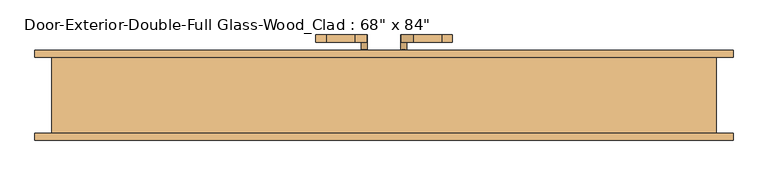
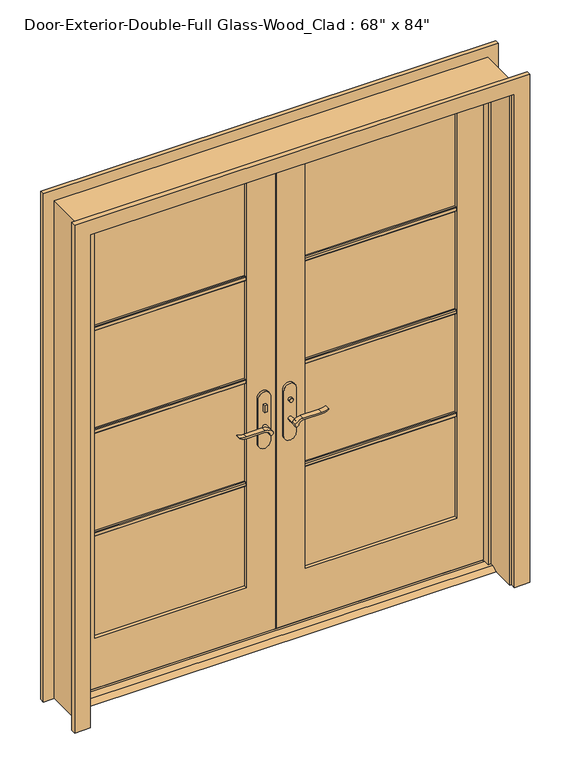
"""IFC4 building model written with IfcOpenShell, lengths in millimetres: door geometry."""

from ifc_helpers import new_model, si_unit, point, frame, frame_2d, origin, place, context, project, spatial, polyline, circle_curve, trimmed, segment, composite_curve, outline, extrude, faceted_brep, source, transform, mapped, element, save


def door_f342fe49(model_context):
    return source(origin(), model_context, "Body", "SolidModel", [
        extrude(outline(polyline([(19.05, 12.7), (53.975, 12.7), (79.375, 0.0), (-6.35, 0.0), (19.05, 12.7)])), frame((-863.6, 0.0, 0.0), z_axis=(1.0, 0.0, 0.0), x_axis=(0.0, 1.0, 0.0)), (0.0, 0.0, 1.0), 1727.2),
        extrude(outline(polyline([(-47.4019111, 43.5), (-57.4019111, 43.5), (-57.4019111, 53.5), (-47.4019111, 53.5), (-47.4019111, 43.5)])), frame((0.0, 0.0, 981.9), z_axis=(0.0, 0.0, 1.0), x_axis=(1.0, 0.0, 0.0)), (0.0, 0.0, 1.0), 30.0),
        extrude(outline(composite_curve([segment(trimmed(circle_curve(frame_2d((996.9, -52.4019111)), 8.0), [point((996.9, -60.4019111))], [point((996.9, -44.4019111))], False, "CARTESIAN"), True, "CONTINUOUS"), segment(trimmed(circle_curve(frame_2d((996.9, -52.4019111)), 8.0), [point((996.9, -44.4019111))], [point((996.9, -60.4019111))], False, "CARTESIAN"), True, "CONTINUOUS")], self_intersect=False)), frame((0.0, 108.425, 0.0), z_axis=(0.0, 1.0, 0.0), x_axis=(0.0, 0.0, 1.0)), (0.0, 0.0, 1.0), 10.0),
        extrude(outline(composite_curve([segment(trimmed(circle_curve(frame_2d((897.1555521, -76.0694241)), 37.2832219), [point((919.0523287, -45.8937749))], [point((934.4, -77.7693445))], False, "CARTESIAN"), True, "CONTINUOUS"), segment(polyline([(934.4, -77.7693445), (934.4, -154.045502)]), True, "CONTINUOUS"), segment(trimmed(circle_curve(frame_2d((1017.6850638, -153.9791202)), 83.2850902), [point((934.4, -154.045502))], [point((939.4, -182.4019111))], True, "CARTESIAN"), True, "CONTINUOUS"), segment(polyline([(939.4, -182.4019111), (936.6135558, -182.4019111)]), True, "CONTINUOUS"), segment(trimmed(circle_curve(frame_2d((986.6709207, -150.4622499)), 59.3791355), [point((936.6135558, -182.4019111))], [point((927.4, -154.045502))], False, "CARTESIAN"), True, "CONTINUOUS"), segment(polyline([(927.4, -154.045502), (927.4, -77.7881013)]), True, "CONTINUOUS"), segment(trimmed(circle_curve(frame_2d((909.2738613, -77.7881013)), 18.1261387), [point((927.4, -77.7881013))], [point((914.4, -60.4019111))], True, "CARTESIAN"), True, "CONTINUOUS"), segment(trimmed(circle_curve(frame_2d((914.4, -52.4019111)), 8.0), [point((914.4, -60.4019111))], [point((919.0523287, -45.8937749))], False, "CARTESIAN"), True, "CONTINUOUS")], self_intersect=False)), frame((0.0, 3.5, 0.0), z_axis=(0.0, 1.0, 0.0), x_axis=(0.0, 0.0, 1.0)), (0.0, 0.0, 1.0), 20.0),
        extrude(outline(composite_curve([segment(trimmed(circle_curve(frame_2d((914.4, -52.4019111)), 8.0), [point((914.3999903, -60.4019111))], [point((919.0523287, -45.8937749))], False, "CARTESIAN"), True, "CONTINUOUS"), segment(trimmed(circle_curve(frame_2d((897.1555521, -76.0694241)), 37.2832219), [point((919.0523287, -45.8937749))], [point((934.4, -77.7693445))], False, "CARTESIAN"), True, "CONTINUOUS"), segment(polyline([(934.4, -77.7693445), (934.4, -154.045502)]), True, "CONTINUOUS"), segment(trimmed(circle_curve(frame_2d((1017.6850638, -153.9791202)), 83.2850902), [point((934.4, -154.045502))], [point((939.4, -182.4019111))], True, "CARTESIAN"), True, "CONTINUOUS"), segment(polyline([(939.4, -182.4019111), (936.6135558, -182.4019111)]), True, "CONTINUOUS"), segment(trimmed(circle_curve(frame_2d((986.6709207, -150.4622499)), 59.3791355), [point((936.6135558, -182.4019111))], [point((927.4, -154.045502))], False, "CARTESIAN"), True, "CONTINUOUS"), segment(polyline([(927.4, -154.045502), (927.4, -77.788099)]), True, "CONTINUOUS"), segment(trimmed(circle_curve(frame_2d((909.2738682, -77.788099)), 18.1261318), [point((927.4, -77.788099))], [point((914.3999903, -60.4019111))], True, "CARTESIAN"), True, "CONTINUOUS")], self_intersect=False)), frame((0.0, 138.425, 0.0), z_axis=(0.0, 1.0, 0.0), x_axis=(0.0, 0.0, 1.0)), (0.0, 0.0, 1.0), 20.0),
        extrude(outline(composite_curve([segment(trimmed(circle_curve(frame_2d((914.4, -52.4019111)), 8.0), [point((914.4, -60.4019111))], [point((914.4, -44.4019111))], False, "CARTESIAN"), True, "CONTINUOUS"), segment(trimmed(circle_curve(frame_2d((914.4, -52.4019111)), 8.0), [point((914.4, -44.4019111))], [point((914.4, -60.4019111))], False, "CARTESIAN"), True, "CONTINUOUS")], self_intersect=False)), frame((0.0, 23.5, 0.0), z_axis=(0.0, 1.0, 0.0), x_axis=(0.0, 0.0, 1.0)), (0.0, 0.0, 1.0), 30.0),
        extrude(outline(composite_curve([segment(trimmed(circle_curve(frame_2d((914.4, -52.4019111)), 8.0), [point((914.4, -60.4019111))], [point((914.4, -44.4019111))], False, "CARTESIAN"), True, "CONTINUOUS"), segment(trimmed(circle_curve(frame_2d((914.4, -52.4019111)), 8.0), [point((914.4, -44.4019111))], [point((914.4, -60.4019111))], False, "CARTESIAN"), True, "CONTINUOUS")], self_intersect=False)), frame((0.0, 108.425, 0.0), z_axis=(0.0, 1.0, 0.0), x_axis=(0.0, 0.0, 1.0)), (0.0, 0.0, 1.0), 30.0),
        extrude(outline(composite_curve([segment(polyline([(844.4, -27.4019111), (1039.4, -27.4019111)]), True, "CONTINUOUS"), segment(trimmed(circle_curve(frame_2d((1039.4, -52.4019111)), 25.0), [point((1039.4, -27.4019111))], [point((1039.4, -77.4019111))], False, "CARTESIAN"), True, "CONTINUOUS"), segment(polyline([(1039.4, -77.4019111), (844.4, -77.4019111)]), True, "CONTINUOUS"), segment(trimmed(circle_curve(frame_2d((844.4, -52.4019111)), 25.0), [point((844.4, -77.4019111))], [point((844.4, -27.4019111))], False, "CARTESIAN"), True, "CONTINUOUS")], self_intersect=False)), frame((0.0, 53.5, 0.0), z_axis=(0.0, 1.0, 0.0), x_axis=(0.0, 0.0, 1.0)), (0.0, 0.0, 1.0), 10.0),
        extrude(outline(composite_curve([segment(polyline([(844.4, -27.4019111), (1039.4, -27.4019111)]), True, "CONTINUOUS"), segment(trimmed(circle_curve(frame_2d((1039.4, -52.4019111)), 25.0), [point((1039.4, -27.4019111))], [point((1039.4, -77.4019111))], False, "CARTESIAN"), True, "CONTINUOUS"), segment(polyline([(1039.4, -77.4019111), (844.4, -77.4019111)]), True, "CONTINUOUS"), segment(trimmed(circle_curve(frame_2d((844.4, -52.4019111)), 25.0), [point((844.4, -77.4019111))], [point((844.4, -27.4019111))], False, "CARTESIAN"), True, "CONTINUOUS")], self_intersect=False)), frame((0.0, 98.425, 0.0), z_axis=(0.0, 1.0, 0.0), x_axis=(0.0, 0.0, 1.0)), (0.0, 0.0, 1.0), 10.0),
        extrude(outline(polyline([(47.3875, 118.425), (57.3875, 118.425), (57.3875, 108.425), (47.3875, 108.425), (47.3875, 118.425)])), frame((0.0, 0.0, 981.9), z_axis=(0.0, 0.0, 1.0), x_axis=(1.0, 0.0, 0.0)), (0.0, 0.0, 1.0), 30.0),
        extrude(outline(composite_curve([segment(trimmed(circle_curve(frame_2d((996.9, 52.3875)), 8.0), [point((996.9, 60.3875))], [point((996.9, 44.3875))], False, "CARTESIAN"), True, "CONTINUOUS"), segment(trimmed(circle_curve(frame_2d((996.9, 52.3875)), 8.0), [point((996.9, 44.3875))], [point((996.9, 60.3875))], False, "CARTESIAN"), True, "CONTINUOUS")], self_intersect=False)), frame((0.0, 43.5, 0.0), z_axis=(0.0, 1.0, 0.0), x_axis=(0.0, 0.0, 1.0)), (0.0, 0.0, 1.0), 10.0),
        extrude(outline(composite_curve([segment(trimmed(circle_curve(frame_2d((914.4, 52.3875)), 8.0), [point((919.0523287, 45.8793637))], [point((914.4, 60.3875))], False, "CARTESIAN"), True, "CONTINUOUS"), segment(trimmed(circle_curve(frame_2d((909.2738613, 77.7736901)), 18.1261387), [point((914.4, 60.3875))], [point((927.4, 77.7736901))], True, "CARTESIAN"), True, "CONTINUOUS"), segment(polyline([(927.4, 77.7736901), (927.4, 154.0310909)]), True, "CONTINUOUS"), segment(trimmed(circle_curve(frame_2d((986.6709207, 150.4478388)), 59.3791355), [point((927.4, 154.0310909))], [point((936.6135558, 182.3875))], False, "CARTESIAN"), True, "CONTINUOUS"), segment(polyline([(936.6135558, 182.3875), (939.4, 182.3875)]), True, "CONTINUOUS"), segment(trimmed(circle_curve(frame_2d((1017.6850638, 153.9647091)), 83.2850902), [point((939.4, 182.3875))], [point((934.4, 154.0310909))], True, "CARTESIAN"), True, "CONTINUOUS"), segment(polyline([(934.4, 154.0310909), (934.4, 77.7549333)]), True, "CONTINUOUS"), segment(trimmed(circle_curve(frame_2d((897.1555521, 76.0550129)), 37.2832219), [point((934.4, 77.7549333))], [point((919.0523287, 45.8793637))], False, "CARTESIAN"), True, "CONTINUOUS")], self_intersect=False)), frame((0.0, 138.425, 0.0), z_axis=(0.0, 1.0, 0.0), x_axis=(0.0, 0.0, 1.0)), (0.0, 0.0, 1.0), 20.0),
        extrude(outline(composite_curve([segment(trimmed(circle_curve(frame_2d((909.2738682, 77.7736878)), 18.1261318), [point((914.3999903, 60.3875))], [point((927.4, 77.7736878))], True, "CARTESIAN"), True, "CONTINUOUS"), segment(polyline([(927.4, 77.7736878), (927.4, 154.0310909)]), True, "CONTINUOUS"), segment(trimmed(circle_curve(frame_2d((986.6709207, 150.4478388)), 59.3791355), [point((927.4, 154.0310909))], [point((936.6135558, 182.3875))], False, "CARTESIAN"), True, "CONTINUOUS"), segment(polyline([(936.6135558, 182.3875), (939.4, 182.3875)]), True, "CONTINUOUS"), segment(trimmed(circle_curve(frame_2d((1017.6850638, 153.9647091)), 83.2850902), [point((939.4, 182.3875))], [point((934.4, 154.0310909))], True, "CARTESIAN"), True, "CONTINUOUS"), segment(polyline([(934.4, 154.0310909), (934.4, 77.7549333)]), True, "CONTINUOUS"), segment(trimmed(circle_curve(frame_2d((897.1555521, 76.0550129)), 37.2832219), [point((934.4, 77.7549333))], [point((919.0523287, 45.8793637))], False, "CARTESIAN"), True, "CONTINUOUS"), segment(trimmed(circle_curve(frame_2d((914.4, 52.3875)), 8.0), [point((919.0523287, 45.8793637))], [point((914.3999903, 60.3875))], False, "CARTESIAN"), True, "CONTINUOUS")], self_intersect=False)), frame((0.0, 3.5, 0.0), z_axis=(0.0, 1.0, 0.0), x_axis=(0.0, 0.0, 1.0)), (0.0, 0.0, 1.0), 20.0),
        extrude(outline(composite_curve([segment(trimmed(circle_curve(frame_2d((914.4, 52.3875)), 8.0), [point((914.4, 60.3875))], [point((914.4, 44.3875))], False, "CARTESIAN"), True, "CONTINUOUS"), segment(trimmed(circle_curve(frame_2d((914.4, 52.3875)), 8.0), [point((914.4, 44.3875))], [point((914.4, 60.3875))], False, "CARTESIAN"), True, "CONTINUOUS")], self_intersect=False)), frame((0.0, 108.425, 0.0), z_axis=(0.0, 1.0, 0.0), x_axis=(0.0, 0.0, 1.0)), (0.0, 0.0, 1.0), 30.0),
        extrude(outline(composite_curve([segment(trimmed(circle_curve(frame_2d((914.4, 52.3875)), 8.0), [point((914.4, 60.3875))], [point((914.4, 44.3875))], False, "CARTESIAN"), True, "CONTINUOUS"), segment(trimmed(circle_curve(frame_2d((914.4, 52.3875)), 8.0), [point((914.4, 44.3875))], [point((914.4, 60.3875))], False, "CARTESIAN"), True, "CONTINUOUS")], self_intersect=False)), frame((0.0, 23.5, 0.0), z_axis=(0.0, 1.0, 0.0), x_axis=(0.0, 0.0, 1.0)), (0.0, 0.0, 1.0), 30.0),
        extrude(outline(composite_curve([segment(trimmed(circle_curve(frame_2d((844.4, 52.3875)), 25.0), [point((844.4, 27.3875))], [point((844.4, 77.3875))], False, "CARTESIAN"), True, "CONTINUOUS"), segment(polyline([(844.4, 77.3875), (1039.4, 77.3875)]), True, "CONTINUOUS"), segment(trimmed(circle_curve(frame_2d((1039.4, 52.3875)), 25.0), [point((1039.4, 77.3875))], [point((1039.4, 27.3875))], False, "CARTESIAN"), True, "CONTINUOUS"), segment(polyline([(1039.4, 27.3875), (844.4, 27.3875)]), True, "CONTINUOUS")], self_intersect=False)), frame((0.0, 98.425, 0.0), z_axis=(0.0, 1.0, 0.0), x_axis=(0.0, 0.0, 1.0)), (0.0, 0.0, 1.0), 10.0),
        extrude(outline(composite_curve([segment(trimmed(circle_curve(frame_2d((844.4, 52.3875)), 25.0), [point((844.4, 27.3875))], [point((844.4, 77.3875))], False, "CARTESIAN"), True, "CONTINUOUS"), segment(polyline([(844.4, 77.3875), (1039.4, 77.3875)]), True, "CONTINUOUS"), segment(trimmed(circle_curve(frame_2d((1039.4, 52.3875)), 25.0), [point((1039.4, 77.3875))], [point((1039.4, 27.3875))], False, "CARTESIAN"), True, "CONTINUOUS"), segment(polyline([(1039.4, 27.3875), (844.4, 27.3875)]), True, "CONTINUOUS")], self_intersect=False)), frame((0.0, 53.5, 0.0), z_axis=(0.0, 1.0, 0.0), x_axis=(0.0, 0.0, 1.0)), (0.0, 0.0, 1.0), 10.0),
        extrude(outline(polyline([(77.47, 1578.371875), (77.47, 1559.321875), (71.12, 1559.321875), (67.945, 1562.496875), (67.945, 1575.196875), (71.12, 1578.371875), (77.47, 1578.371875)])), frame((120.65, 0.0, 0.0), z_axis=(1.0, 0.0, 0.0), x_axis=(0.0, 1.0, 0.0)), (0.0, 0.0, 1.0), 622.3),
        extrude(outline(polyline([(77.47, 1132.68125), (77.47, 1113.63125), (71.12, 1113.63125), (67.945, 1116.80625), (67.945, 1129.50625), (71.12, 1132.68125), (77.47, 1132.68125)])), frame((120.65, 0.0, 0.0), z_axis=(1.0, 0.0, 0.0), x_axis=(0.0, 1.0, 0.0)), (0.0, 0.0, 1.0), 622.3),
        extrude(outline(polyline([(77.47, 686.990625), (77.47, 667.940625), (71.12, 667.940625), (67.945, 671.115625), (67.945, 683.815625), (71.12, 686.990625), (77.47, 686.990625)])), frame((120.65, 0.0, 0.0), z_axis=(1.0, 0.0, 0.0), x_axis=(0.0, 1.0, 0.0)), (0.0, 0.0, 1.0), 622.3),
        extrude(outline(polyline([(84.455, 1578.371875), (90.805, 1578.371875), (93.98, 1575.196875), (93.98, 1562.496875), (90.805, 1559.321875), (84.455, 1559.321875), (84.455, 1578.371875)])), frame((-742.95, 0.0, 0.0), z_axis=(1.0, 0.0, 0.0), x_axis=(0.0, 1.0, 0.0)), (0.0, 0.0, 1.0), 622.3),
        extrude(outline(polyline([(84.455, 1132.68125), (90.805, 1132.68125), (93.98, 1129.50625), (93.98, 1116.80625), (90.805, 1113.63125), (84.455, 1113.63125), (84.455, 1132.68125)])), frame((-742.95, 0.0, 0.0), z_axis=(1.0, 0.0, 0.0), x_axis=(0.0, 1.0, 0.0)), (0.0, 0.0, 1.0), 622.3),
        extrude(outline(polyline([(84.455, 686.990625), (90.805, 686.990625), (93.98, 683.815625), (93.98, 671.115625), (90.805, 667.940625), (84.455, 667.940625), (84.455, 686.990625)])), frame((-742.95, 0.0, 0.0), z_axis=(1.0, 0.0, 0.0), x_axis=(0.0, 1.0, 0.0)), (0.0, 0.0, 1.0), 622.3),
        extrude(outline(polyline([(84.455, 1578.371875), (90.805, 1578.371875), (93.98, 1575.196875), (93.98, 1562.496875), (90.805, 1559.321875), (84.455, 1559.321875), (84.455, 1578.371875)])), frame((120.65, 0.0, 0.0), z_axis=(1.0, 0.0, 0.0), x_axis=(0.0, 1.0, 0.0)), (0.0, 0.0, 1.0), 622.3),
        extrude(outline(polyline([(84.455, 1132.68125), (90.805, 1132.68125), (93.98, 1129.50625), (93.98, 1116.80625), (90.805, 1113.63125), (84.455, 1113.63125), (84.455, 1132.68125)])), frame((120.65, 0.0, 0.0), z_axis=(1.0, 0.0, 0.0), x_axis=(0.0, 1.0, 0.0)), (0.0, 0.0, 1.0), 622.3),
        extrude(outline(polyline([(84.455, 686.990625), (90.805, 686.990625), (93.98, 683.815625), (93.98, 671.115625), (90.805, 667.940625), (84.455, 667.940625), (84.455, 686.990625)])), frame((120.65, 0.0, 0.0), z_axis=(1.0, 0.0, 0.0), x_axis=(0.0, 1.0, 0.0)), (0.0, 0.0, 1.0), 622.3),
        extrude(outline(polyline([(77.47, 1578.371875), (77.47, 1559.321875), (71.12, 1559.321875), (67.945, 1562.496875), (67.945, 1575.196875), (71.12, 1578.371875), (77.47, 1578.371875)])), frame((-742.95, 0.0, 0.0), z_axis=(1.0, 0.0, 0.0), x_axis=(0.0, 1.0, 0.0)), (0.0, 0.0, 1.0), 622.3),
        extrude(outline(polyline([(77.47, 1132.68125), (77.47, 1113.63125), (71.12, 1113.63125), (67.945, 1116.80625), (67.945, 1129.50625), (71.12, 1132.68125), (77.47, 1132.68125)])), frame((-742.95, 0.0, 0.0), z_axis=(1.0, 0.0, 0.0), x_axis=(0.0, 1.0, 0.0)), (0.0, 0.0, 1.0), 622.3),
        extrude(outline(polyline([(77.47, 686.990625), (77.47, 667.940625), (71.12, 667.940625), (67.945, 671.115625), (67.945, 683.815625), (71.12, 686.990625), (77.47, 686.990625)])), frame((-742.95, 0.0, 0.0), z_axis=(1.0, 0.0, 0.0), x_axis=(0.0, 1.0, 0.0)), (0.0, 0.0, 1.0), 622.3),
        extrude(outline(polyline([(0.0, 869.95), (0.0, 933.45), (2203.45, 933.45), (2203.45, -933.45), (0.0, -933.45), (0.0, -869.95), (2139.95, -869.95), (2139.95, 869.95), (0.0, 869.95)])), frame((0.0, 98.425, 0.0), z_axis=(0.0, 1.0, 0.0), x_axis=(0.0, 0.0, 1.0)), (0.0, 0.0, 1.0), 19.05),
        extrude(outline(polyline([(0.0, 869.95), (0.0, 933.45), (2203.45, 933.45), (2203.45, -933.45), (0.0, -933.45), (0.0, -869.95), (2139.95, -869.95), (2139.95, 869.95), (0.0, 869.95)])), frame((0.0, -123.825, 0.0), z_axis=(0.0, 1.0, 0.0), x_axis=(0.0, 0.0, 1.0)), (0.0, 0.0, 1.0), 19.05),
        extrude(outline(polyline([(12.7, 863.6), (2133.6, 863.6), (2133.6, 1.5875), (12.7, 1.5875), (12.7, 863.6)]), holes=[polyline([(2014.5375, 120.65), (2014.5375, 742.95), (231.775, 742.95), (231.775, 120.65), (2014.5375, 120.65)])]), frame((0.0, 63.5, 0.0), z_axis=(0.0, 1.0, 0.0), x_axis=(0.0, 0.0, 1.0)), (0.0, 0.0, 1.0), 34.925),
        extrude(outline(polyline([(2133.6, -863.6), (12.7, -863.6), (12.7, -1.6019111), (2133.6, -1.6019111), (2133.6, -863.6)]), holes=[polyline([(231.775, -742.95), (2014.5375, -742.95), (2014.5375, -120.65), (231.775, -120.65), (231.775, -742.95)])]), frame((0.0, 63.5, 0.0), z_axis=(0.0, 1.0, 0.0), x_axis=(0.0, 0.0, 1.0)), (0.0, 0.0, 1.0), 34.925),
        faceted_brep([(889.0, 98.425, 0.0), (889.0, -104.775, 0.0), (863.6, -104.775, 0.0), (863.6, 28.575, 0.0), (850.9, 28.575, 0.0), (850.9, 63.5, 0.0), (863.6, 63.5, 0.0), (863.6, 98.425, 0.0), (889.0, 98.425, 2159.0), (889.0, -104.775, 2159.0), (-889.0, -104.775, 2159.0), (-889.0, -104.775, 0.0), (-863.6, -104.775, 0.0), (-863.6, -104.775, 2133.6), (863.6, -104.775, 2133.6), (863.6, 28.575, 2133.6), (-863.6, 28.575, 2133.6), (-863.6, 28.575, 0.0), (-850.9, 28.575, 0.0), (-850.9, 28.575, 2120.9), (850.9, 28.575, 2120.9), (850.9, 63.5, 2120.9), (1.5875, 63.5, 2120.9), (-1.6019111, 63.5, 2120.9), (-850.9, 63.5, 2120.9), (-850.9, 63.5, 0.0), (-863.6, 63.5, 0.0), (-863.6, 63.5, 2133.6), (-1.6019111, 63.5, 2133.6), (1.5875, 63.5, 2133.6), (863.6, 63.5, 2133.6), (863.6, 98.425, 2133.6), (1.5875, 98.425, 2133.6), (-1.6019111, 98.425, 2133.6), (-863.6, 98.425, 2133.6), (-863.6, 98.425, 0.0), (-889.0, 98.425, 0.0), (-889.0, 98.425, 2159.0)], [[[0, 1, 2, 3, 4, 5, 6, 7]], [[1, 0, 8, 9]], [[2, 1, 9, 10, 11, 12, 13, 14]], [[3, 2, 14, 15]], [[4, 3, 15, 16, 17, 18, 19, 20]], [[5, 4, 20, 21]], [[6, 5, 21, 22, 23, 24, 25, 26, 27, 28, 29, 30]], [[7, 6, 30, 31]], [[0, 7, 31, 32, 33, 34, 35, 36, 37, 8]], [[9, 8, 37, 10]], [[14, 13, 16, 15]], [[20, 19, 24, 23, 22, 21]], [[31, 30, 29, 28, 27, 34, 33, 32]], [[12, 11, 36, 35, 26, 25, 18, 17]], [[11, 10, 37, 36]], [[13, 12, 17, 16]], [[19, 18, 25, 24]], [[27, 26, 35, 34]]]),
        extrude(outline(polyline([(742.95, 77.47), (120.65, 77.47), (120.65, 84.455), (742.95, 84.455), (742.95, 77.47)])), frame((0.0, 0.0, 231.775), z_axis=(0.0, 0.0, 1.0), x_axis=(1.0, 0.0, 0.0)), (0.0, 0.0, 1.0), 1782.7625),
        extrude(outline(polyline([(-120.65, 77.47), (-742.95, 77.47), (-742.95, 84.455), (-120.65, 84.455), (-120.65, 77.47)])), frame((0.0, 0.0, 231.775), z_axis=(0.0, 0.0, 1.0), x_axis=(1.0, 0.0, 0.0)), (0.0, 0.0, 1.0), 1782.7625),
    ])


if __name__ == "__main__":
    model = new_model("IFC4")
    model_context = context("Model", 3, world=origin())
    ifc_project = project(units=[si_unit("LENGTHUNIT", "METRE", prefix="MILLI")], contexts=[model_context])
    site = spatial("IfcSite", under=ifc_project)
    building = spatial("IfcBuilding", under=site)
    placement = place(None, origin())
    door_shape = door_f342fe49(model_context)
    element("IfcDoor", 1, ObjectType="Door-Exterior-Double-Full Glass-Wood_Clad : 68\" x 84\"", at=placement, inside=building, context=model_context, shape_type="MappedRepresentation", body=[
        mapped(door_shape, transform((0.0, 0.0, 0.0), x_axis=(1.0, 0.0, 0.0), y_axis=(0.0, 1.0, 0.0), z_axis=(0.0, 0.0, 1.0))),
    ])
    save(model, "model.ifc")

# Revit data of these elements
# Type "Door-Exterior-Double-Full Glass-Wood_Clad : 68\" x 84\""
#   Type Mark = "11"
#   Assembly Code = "B2030100"
#   Analytic Construction = "French door, wood frame with double glass"
#   Top Rail = 0.390625 ft
#   Threshold Offset [instance default] = 0.041667 ft
#   Thickness = 0.114583 ft
#   Thermal Resistance (R) = 1.9158 (h·ft²·°F)/BTU
#   Swing Angle [instance default] = 90.00°
#   Stiles = 0.395833 ft
#   Rough Width = 5.833333 ft
#   Rough Height = 7.083333 ft
#   Panel Width = 2.833333 ft
#   Door Offset [instance default] = 0.00 ft
#   Height = 7.00 ft
#   Width = 5.666667 ft
#   Heat Transfer Coefficient (U) = 0.5220 BTU/(h·ft²·°F)
#   Bottom Rail = 0.760417 ft
#   Exterior Trim [instance default] = yes
#   Threshold [instance default] = yes
#   Show Grill [instance default] = yes
#   Function = 1
#   Trim Material = Cherry
#   Threshold Material = Cherry
#   Panel Material = Cherry
#   Glazing = Glass
#   Frame Material = Cherry
#   Door Handle Material = Aluminum
#   Visual Light Transmittance = 0
#   Solar Heat Gain Coefficient = 0
#   Wall Closure = (empty or 0)
#   Construction Type = (empty or 0)
# Element 1 (IfcDoor, "Door-Exterior-Double-Full Glass-Wood_Clad : 68\" x 84\"")
#   Materials on its faces: "Cherry", "Aluminum", "Glass"
# Materials
#   "Cherry": class "Wood", colour RGB 226 177 128, transparency 0, Description = "Prunus Serotina", Cost = 0
#   "Glass": class "Glass", colour RGB 0 128 192, transparency 0.75, Description = "Soda Lime Glass", Cost = 0
#   "Aluminum": class "Metal", colour RGB 244 245 246, transparency 0, Description = "Aluminum 6061", Cost = 0
